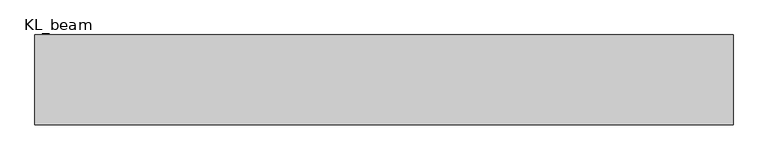
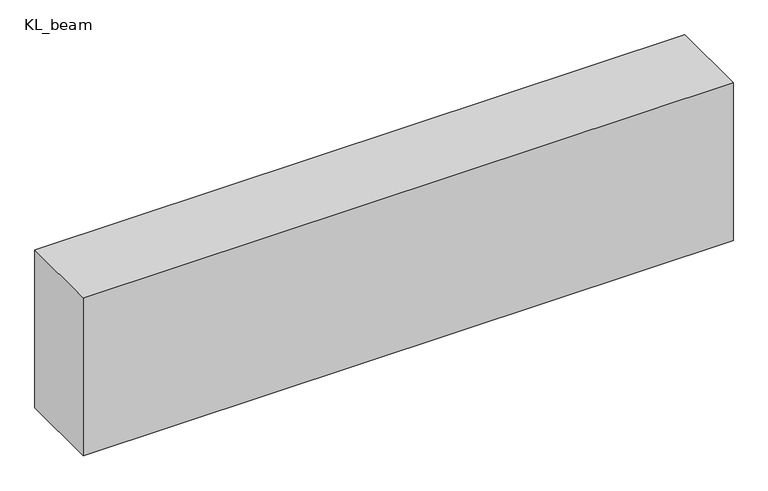
"""IFC4 building model written with IfcOpenShell, lengths in millimetres: beam geometry, 混凝土 - 矩形梁 : KL_beam."""

from ifc_helpers import new_model, si_unit, frame, origin, place, context, project, spatial, polyline, outline, extrude, source, transform, mapped, element, save


def kl_beam_68dd7060(model_context):
    return source(origin(), model_context, "Body", "SweptSolid", [
        extrude(outline(polyline([(1555.0, 200.0), (1555.0, -200.0), (-1555.0, -200.0), (-1555.0, 200.0), (1555.0, 200.0)])), frame((0.0, 0.0, -400.0), z_axis=(0.0, 0.0, 1.0), x_axis=(1.0, 0.0, 0.0)), (0.0, 0.0, 1.0), 800.0),
    ])


if __name__ == "__main__":
    model = new_model("IFC4")
    model_context = context("Model", 3, world=origin())
    ifc_project = project(units=[si_unit("LENGTHUNIT", "METRE", prefix="MILLI")], contexts=[model_context])
    site = spatial("IfcSite", under=ifc_project)
    building = spatial("IfcBuilding", under=site)
    placement = place(None, origin())
    kl_beam_shape = kl_beam_68dd7060(model_context)
    element("IfcBeam", 1, ObjectType="混凝土 - 矩形梁 : KL_beam", at=placement, inside=building, context=model_context, shape_type="MappedRepresentation", body=[
        mapped(kl_beam_shape, transform((0.0, 0.0, 0.0), x_axis=(1.0, 0.0, 0.0), y_axis=(0.0, 1.0, 0.0), z_axis=(0.0, 0.0, 1.0))),
    ])
    save(model, "model.ifc")

# Revit data of these elements
# Type "混凝土 - 矩形梁 : KL_beam"
#   Length [instance default] = 1524 mm
#   b = 400 mm
#   h = 800 mm
#   Structural Material [instance default] = 混凝土 - 现场浇注混凝土
#   Assembly Code = ""
# Element 1 (IfcBeam, "混凝土 - 矩形梁 : KL_beam")
#   Structural Material = none
# Materials
#   "混凝土 - 现场浇注混凝土": class "混凝土", colour RGB 192 192 192, transparency 0
